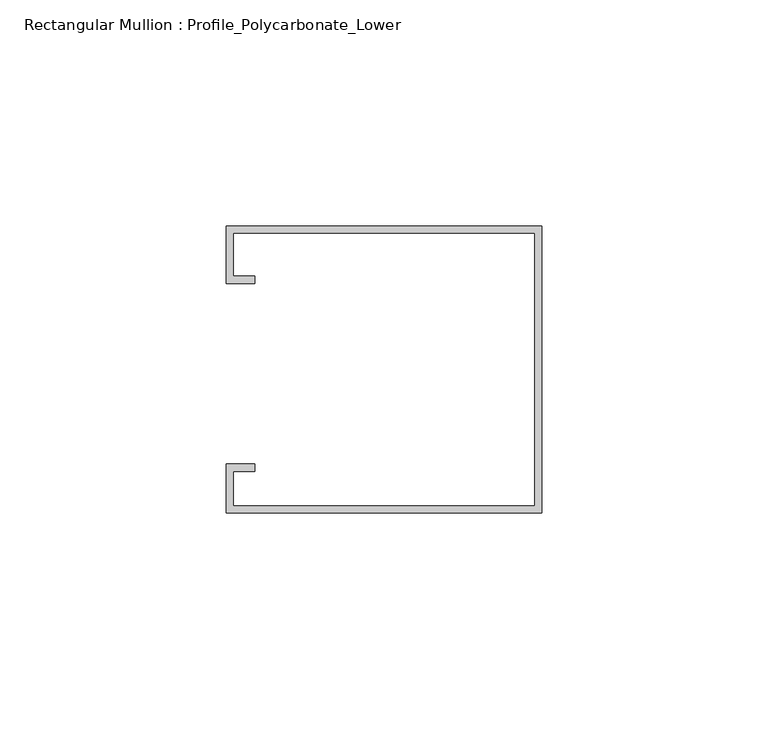
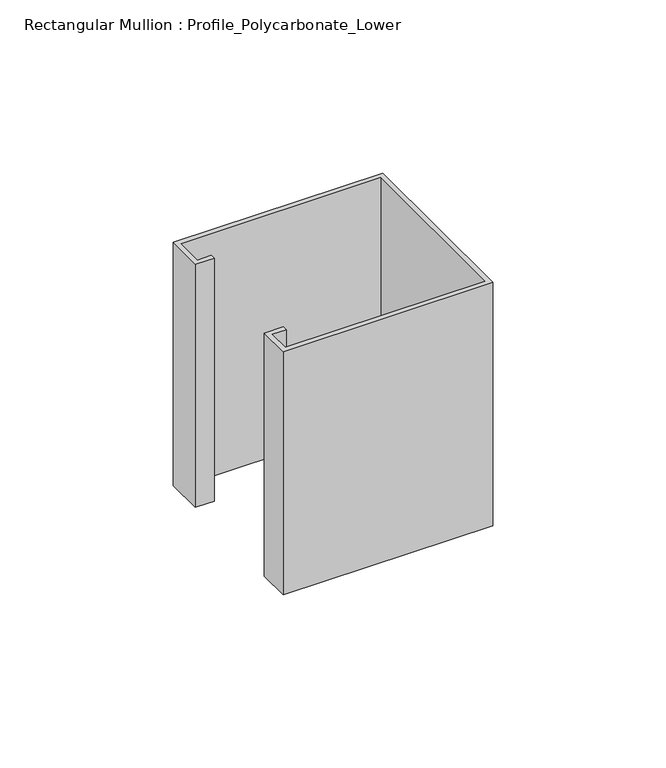
"""IFC4 building model written with IfcOpenShell, lengths in millimetres: member geometry, Rectangular Mullion : Profile_Polycarbonate_Lower."""

from ifc_helpers import new_model, si_unit, frame, origin, place, context, project, spatial, polyline, outline, extrude, source, transform, mapped, element, save


def rectangular_mullion_profile_polycarbonate_lower_ca088a1d(model_context):
    return source(origin(), model_context, "Body", "SweptSolid", [
        extrude(outline(polyline([(0.0, 32.7), (0.0, -30.8), (-69.85, -30.8), (-69.85, -20.0), (-63.5, -20.0), (-63.5, -21.5875), (-68.2625, -21.5875), (-68.2625, -29.2125), (-1.5875, -29.2125), (-1.5875, 31.1125), (-68.2625, 31.1125), (-68.2625, 21.5875), (-63.5, 21.5875), (-63.5, 20.0), (-69.85, 20.0), (-69.85, 32.7), (0.0, 32.7)])), frame((0.0, 0.0, -85.725), z_axis=(0.0, 0.0, 1.0), x_axis=(1.0, 0.0, 0.0)), (0.0, 0.0, 1.0), 85.725),
    ])


if __name__ == "__main__":
    model = new_model("IFC4")
    model_context = context("Model", 3, world=origin())
    ifc_project = project(units=[si_unit("LENGTHUNIT", "METRE", prefix="MILLI")], contexts=[model_context])
    site = spatial("IfcSite", under=ifc_project)
    building = spatial("IfcBuilding", under=site)
    placement = place(None, origin())
    rectangular_mullion_profile_polycarbonate_lower_shape = rectangular_mullion_profile_polycarbonate_lower_ca088a1d(model_context)
    element("IfcMember", 1, ObjectType="Rectangular Mullion : Profile_Polycarbonate_Lower", at=placement, inside=building, context=model_context, shape_type="MappedRepresentation", body=[
        mapped(rectangular_mullion_profile_polycarbonate_lower_shape, transform((0.0, 0.0, 0.0), x_axis=(1.0, 0.0, 0.0), y_axis=(0.0, 1.0, 0.0), z_axis=(0.0, 0.0, 1.0))),
    ])
    save(model, "model.ifc")

# Revit data of these elements
# Type "Rectangular Mullion : Profile_Polycarbonate_Lower"
#   built-in parameter 1007322 = 0.208333 (stored number, unit not read)
#   built-in parameter 1007321 = 0 (stored number, unit not read)
#   built-in parameter 1007320 = 0.00520833 (stored number, unit not read)
# Element 1 (IfcMember, "Rectangular Mullion : Profile_Polycarbonate_Lower")
#   Materials on its faces: "GALVANIZED UNISTRUT P5500, 1 5/8\" X 2 7/16\" OR ALUM. CHANNEL"
# Materials
#   "GALVANIZED UNISTRUT P5500, 1 5/8\" X 2 7/16\" OR ALUM. CHANNEL": class "Metal", colour RGB 244 244 244, transparency 0, Description = "Aluminum 6061", Cost = 0
